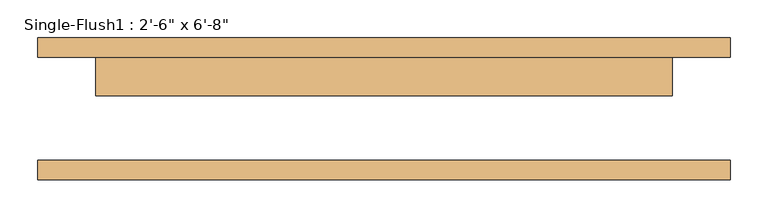
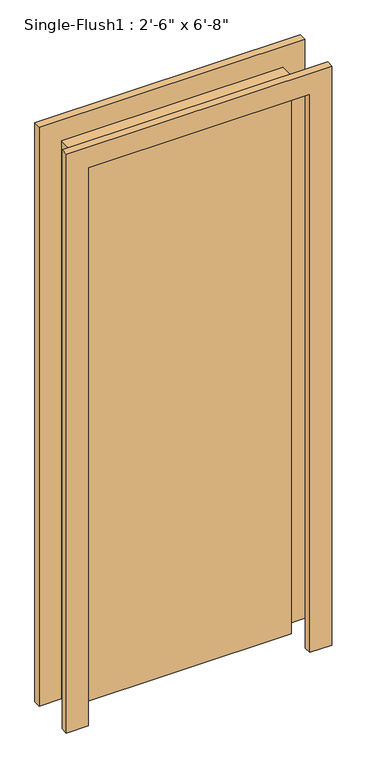
"""IFC4 building model written with IfcOpenShell, lengths in millimetres: door geometry."""

from ifc_helpers import new_model, si_unit, frame, origin, origin_with_axes, place, context, project, spatial, polyline, outline, extrude, source, transform, mapped, element, save


def door_0b154108(model_context):
    return source(origin(), model_context, "Body", "SweptSolid", [
        extrude(outline(polyline([(2108.2, -457.2), (0.0, -457.2), (0.0, -381.0), (2032.0, -381.0), (2032.0, 381.0), (0.0, 381.0), (0.0, 457.2), (2108.2, 457.2), (2108.2, -457.2)])), frame((0.0, 68.2625, 0.0), z_axis=(0.0, 1.0, 0.0), x_axis=(0.0, 0.0, 1.0)), (0.0, 0.0, 1.0), 25.4),
        extrude(outline(polyline([(2108.2, 457.2), (2108.2, -457.2), (0.0, -457.2), (0.0, -381.0), (2032.0, -381.0), (2032.0, 381.0), (0.0, 381.0), (0.0, 457.2), (2108.2, 457.2)])), frame((0.0, -93.6625, 0.0), z_axis=(0.0, 1.0, 0.0), x_axis=(0.0, 0.0, 1.0)), (0.0, 0.0, 1.0), 25.4),
        extrude(outline(polyline([(381.0, 17.4625), (-381.0, 17.4625), (-381.0, 68.2625), (381.0, 68.2625), (381.0, 17.4625)])), origin_with_axes(), (0.0, 0.0, 1.0), 2032.0),
    ])


if __name__ == "__main__":
    model = new_model("IFC4")
    model_context = context("Model", 3, world=origin())
    ifc_project = project(units=[si_unit("LENGTHUNIT", "METRE", prefix="MILLI")], contexts=[model_context])
    site = spatial("IfcSite", under=ifc_project)
    building = spatial("IfcBuilding", under=site)
    placement = place(None, origin())
    door_shape = door_0b154108(model_context)
    element("IfcDoor", 1, ObjectType="Single-Flush1 : 2'-6\" x 6'-8\"", at=placement, inside=building, context=model_context, shape_type="MappedRepresentation", body=[
        mapped(door_shape, transform((0.0, 0.0, 0.0), x_axis=(1.0, 0.0, 0.0), y_axis=(0.0, 1.0, 0.0), z_axis=(0.0, 0.0, 1.0))),
    ])
    save(model, "model.ifc")

# Revit data of these elements
# Type "Single-Flush1 : 2'-6\" x 6'-8\""
#   Type Mark = "D6"
#   Construction Type Id = "MDOOR"
#   Assembly Code = "C1020"
#   Analytic Construction = "Metal"
#   Thickness = 0' - 2"
#   Heat Transfer Coefficient (U) = 3.7021 W/(m²·K)
#   Height = 6' - 8"
#   Trim Projection Ext = 0' - 1"
#   Trim Projection Int = 0' - 1"
#   Trim Width = 0' - 3"
#   Width = 2' - 6"
#   Door Material = Door - Panel
#   Frame Material = Door - Frame
#   Visual Light Transmittance = 0
#   Solar Heat Gain Coefficient = 0
#   Function = (empty or 0)
#   Wall Closure = (empty or 0)
# Element 1 (IfcDoor, "Single-Flush1 : 2'-6\" x 6'-8\"")
#   Materials on its faces: "Door - Frame", "Door - Panel"
# Materials
#   "Door - Panel": class "Wood", colour RGB 210 159 95, transparency 0, Cost = 0
#   "Door - Frame": class "Miscellaneous", colour RGB 118 70 51, transparency 0, Cost = 0
